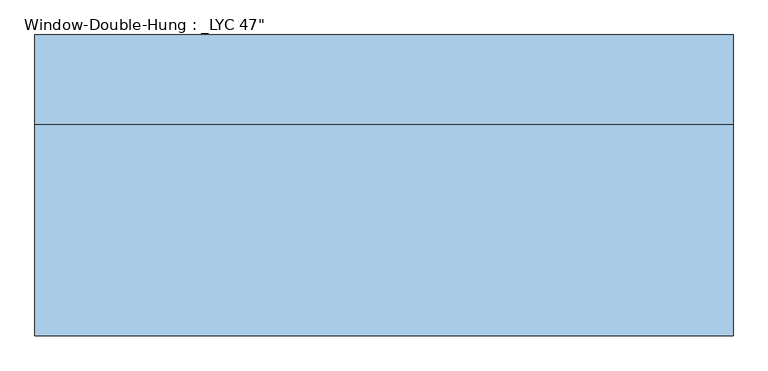
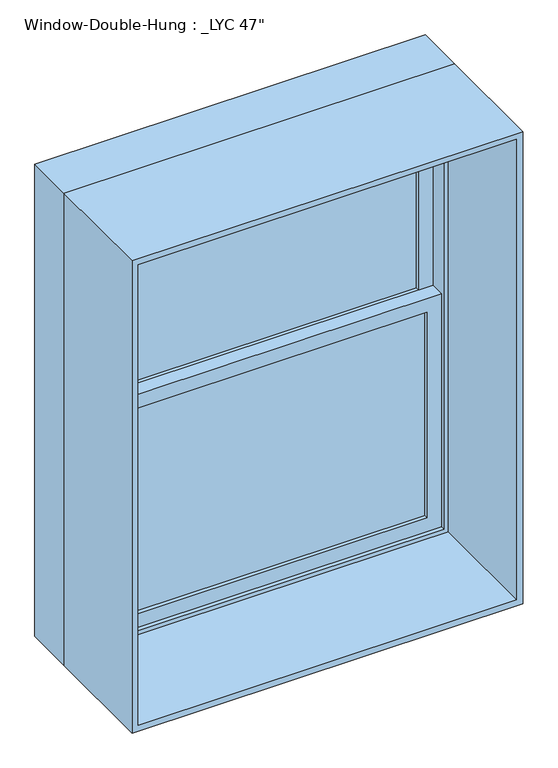
"""IFC4 building model written with IfcOpenShell, lengths in millimetres: window geometry."""

from ifc_helpers import new_model, si_unit, frame, origin, place, context, project, spatial, polyline, outline, extrude, source, transform, mapped, element, save


def window_c164e1cd(model_context):
    return source(origin(), model_context, "Body", "SweptSolid", [
        extrude(outline(polyline([(520.7, 158.75), (520.7, 152.4), (-520.7, 152.4), (-520.7, 158.75), (520.7, 158.75)])), frame((0.0, 0.0, 990.6), z_axis=(0.0, 0.0, 1.0), x_axis=(1.0, 0.0, 0.0)), (0.0, 0.0, 1.0), 663.575),
        extrude(outline(polyline([(-520.7, 146.05), (520.7, 146.05), (520.7, 139.7), (-520.7, 139.7), (-520.7, 146.05)])), frame((0.0, 0.0, 990.6), z_axis=(0.0, 0.0, 1.0), x_axis=(1.0, 0.0, 0.0)), (0.0, 0.0, 1.0), 663.575),
        extrude(outline(polyline([(520.7, 203.2), (520.7, 196.85), (-520.7, 196.85), (-520.7, 203.2), (520.7, 203.2)])), frame((0.0, 0.0, 1698.625), z_axis=(0.0, 0.0, 1.0), x_axis=(1.0, 0.0, 0.0)), (0.0, 0.0, 1.0), 663.575),
        extrude(outline(polyline([(-520.7, 190.5), (520.7, 190.5), (520.7, 184.15), (-520.7, 184.15), (-520.7, 190.5)])), frame((0.0, 0.0, 1698.625), z_axis=(0.0, 0.0, 1.0), x_axis=(1.0, 0.0, 0.0)), (0.0, 0.0, 1.0), 663.575),
        extrude(outline(polyline([(1698.625, -565.15), (946.15, -565.15), (946.15, 565.15), (1698.625, 565.15), (1698.625, -565.15)]), holes=[polyline([(1654.175, 520.7), (990.6, 520.7), (990.6, -520.7), (1654.175, -520.7), (1654.175, 520.7)])]), frame((0.0, 127.0, 0.0), z_axis=(0.0, 1.0, 0.0), x_axis=(0.0, 0.0, 1.0)), (0.0, 0.0, 1.0), 44.45),
        extrude(outline(polyline([(2406.65, -565.15), (1654.175, -565.15), (1654.175, 565.15), (2406.65, 565.15), (2406.65, -565.15)]), holes=[polyline([(2362.2, 520.7), (1698.625, 520.7), (1698.625, -520.7), (2362.2, -520.7), (2362.2, 520.7)])]), frame((0.0, 171.45, 0.0), z_axis=(0.0, 1.0, 0.0), x_axis=(0.0, 0.0, 1.0)), (0.0, 0.0, 1.0), 44.45),
        extrude(outline(polyline([(2438.4, -596.9), (914.4, -596.9), (914.4, 596.9), (2438.4, 596.9), (2438.4, -596.9)]), holes=[polyline([(2406.65, 565.15), (946.15, 565.15), (946.15, -565.15), (2406.65, -565.15), (2406.65, 565.15)])]), frame((0.0, 114.3, 0.0), z_axis=(0.0, 1.0, 0.0), x_axis=(0.0, 0.0, 1.0)), (0.0, 0.0, 1.0), 152.4),
        extrude(outline(polyline([(2438.4, 596.9), (2438.4, -596.9), (914.4, -596.9), (914.4, 596.9), (2438.4, 596.9)]), holes=[polyline([(2419.35, 577.85), (933.45, 577.85), (933.45, -577.85), (2419.35, -577.85), (2419.35, 577.85)])]), frame((0.0, -247.65, 0.0), z_axis=(0.0, 1.0, 0.0), x_axis=(0.0, 0.0, 1.0)), (0.0, 0.0, 1.0), 361.95),
    ])


if __name__ == "__main__":
    model = new_model("IFC4")
    model_context = context("Model", 3, world=origin())
    ifc_project = project(units=[si_unit("LENGTHUNIT", "METRE", prefix="MILLI")], contexts=[model_context])
    site = spatial("IfcSite", under=ifc_project)
    building = spatial("IfcBuilding", under=site)
    placement = place(None, origin())
    window_shape = window_c164e1cd(model_context)
    element("IfcWindow", 1, ObjectType="Window-Double-Hung : _LYC 47\"", at=placement, inside=building, context=model_context, shape_type="MappedRepresentation", body=[
        mapped(window_shape, transform((0.0, 0.0, 0.0), x_axis=(1.0, 0.0, 0.0), y_axis=(0.0, 1.0, 0.0), z_axis=(0.0, 0.0, 1.0))),
    ])
    save(model, "model.ifc")

# Revit data of these elements
# Type "Window-Double-Hung : _LYC 47\""
#   Type Mark = "26"
#   Fire Rating = "0.5h"
#   Assembly Code = "B2020100"
#   Wall Thickness [instance default] = 0' - 6"
#   Visual Light Transmittance = 0.9
#   Thermal Resistance (R) = 1.8146 (h·ft²·°F)/BTU
#   Solar Heat Gain Coefficient = 0.78
#   Rough Width = 3' - 11 1/2"
#   Rough Height = 5' - 0 1/2"
#   Muntin Width = 3' - 5"
#   Muntin Height = 2' - 2 1/8"
#   Interior Wall Closure [instance default] = 0' - 1 1/2"
#   Heat Transfer Coefficient (U) = 0.6496 BTU/(h·ft²·°F)
#   Frame Extension [instance default] = 0' - 2"
#   Exterior Wall Closure [instance default] = 0' - 0 1/2"
#   Extension Jamb [instance default] = 0' - 0 3/4"
#   Height = 5' - 0"
#   Width = 3' - 11"
#   Window Inset [instance default] = 0' - 0 3/4"
#   Top Muntin Visibility = yes
#   Interior Trim Visibility [instance default] = yes
#   Indicator Visibility [instance default] = yes
#   Exterior Trim Visibility [instance default] = yes
#   Extension Jamb Visibility [instance default] = yes
#   Define Thermal Properties by = 1
#   Bottom Muntin Visibility = yes
#   Muntin Pattern = Muntin Pattern_2x2 : Muntin Pattern_2x2
#   Interior Trim Material = Wood - Stained
#   Interior Trim = Trim-Window-Interior-Flat : Picture Frame
#   Interior Frame Material = Wood - Stained
#   Glass Panel Material = Glass
#   Exterior Trim Material = Clad - White
#   Exterior Trim = Trim-Window-Exterior-Flat : with Sill
#   Exterior Frame Material = Clad - White
#   Construction Type Id = ""
#   Wall Closure = (empty or 0)
#   Analytic Construction = (empty or 0)
# Element 1 (IfcWindow, "Window-Double-Hung : _LYC 47\"")
#   Wall Thickness = 1' - 7 1/2"
#   Extension Jamb = 1' - 2 1/4"
#   Materials on its faces: "Wood - Stained", "Glass", "Clad - White"
# Materials
#   "Wood - Stained": class "Wood", colour RGB 224 178 126, transparency 0, Cost = 0
#   "Glass": class "Unassigned", colour RGB 0 128 192, transparency 0.75
#   "Clad - White": class "Wood", colour RGB 242 242 238, transparency 0, Cost = 0
